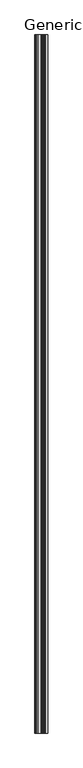
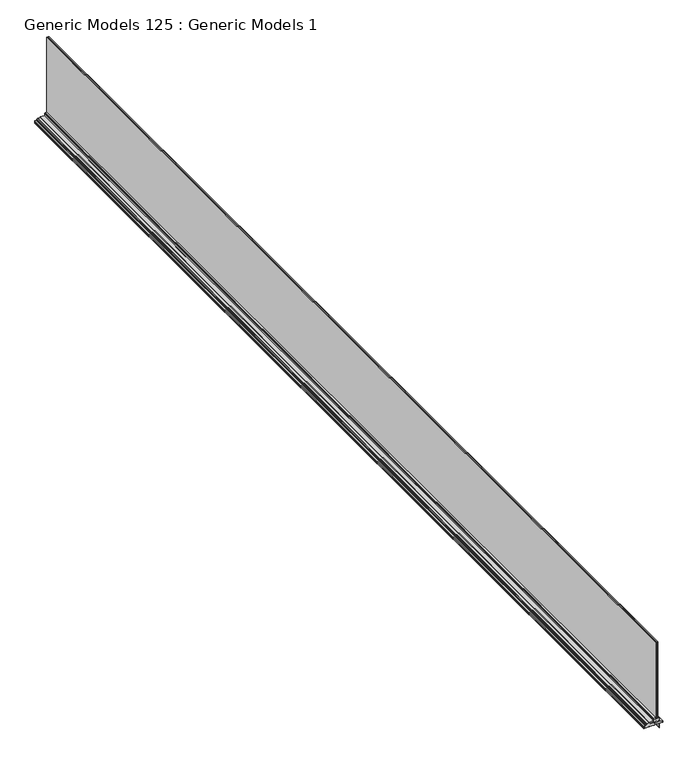
"""IFC4 building model written with IfcOpenShell, lengths in millimetres: proxy geometry, Generic Models 125 : Generic Models 1."""

from ifc_helpers import new_model, si_unit, point, frame, frame_2d, origin, place, context, project, spatial, polyline, circle_curve, trimmed, segment, composite_curve, outline, extrude, source, transform, mapped, element, save


def generic_models_125_generic_models_1_b7fb5337(model_context):
    return source(origin(), model_context, "Body", "SweptSolid", [
        extrude(outline(composite_curve([segment(polyline([(126266.1189906, 4830.4400913), (126266.1189906, 4848.5086347), (126269.2939906, 4848.5086347), (126269.2939906, 4850.7946386), (126266.1189906, 4850.7946386), (126266.1189906, 4868.3023877), (126269.2939906, 4868.3023877), (126269.2939906, 4870.5883916), (126266.1189906, 4870.5883916), (126266.1189906, 4887.6154913), (126268.2017906, 4887.6154913), (126268.2017906, 4890.7904913), (126266.1189906, 4890.7904913), (126266.1189906, 4907.8898738), (126269.2939906, 4907.8898738), (126269.2939906, 4910.1758738), (126266.1189906, 4910.1758738), (126266.1189906, 4946.6450416), (126230.747103, 4946.6450416)]), True, "CONTINUOUS"), segment(trimmed(circle_curve(frame_2d((126230.7494439, 4947.3435419)), 0.6985041), [point((126230.747103, 4946.6450416))], [point((126230.7519036, 4948.0420416))], False, "CARTESIAN"), True, "CONTINUOUS"), segment(polyline([(126230.7519036, 4948.0420416), (126266.1189906, 4948.0420416), (126266.1189906, 4972.929876), (126267.5159906, 4972.929876), (126267.5159906, 4966.579876), (126269.8019906, 4966.579876), (126269.8019906, 4974.4834416), (126278.7334139, 4974.4834416), (126281.1557838, 4946.6196416), (126281.1557838, 4911.6692416), (126286.0325764, 4911.6692416), (126286.0325764, 4907.6561145), (126279.6136368, 4907.6561145), (126279.6136368, 4905.6748401), (126287.5638299, 4905.6748401), (126287.5638299, 4897.2675044), (126288.5036264, 4897.2675044), (126288.5036264, 4879.7415044), (126290.7896264, 4879.7415044), (126290.7896264, 4897.2675044), (126299.4764264, 4897.2675044), (126299.4764264, 4900.3154773), (126302.6514264, 4900.3154773), (126302.6514264, 4870.9022533), (126296.3195939, 4870.9022533), (126296.3195939, 4851.8522533), (126293.9319974, 4851.8522533), (126293.9319974, 4850.2520602), (126290.7569974, 4846.3150913), (126290.7569974, 4844.7148982), (126286.7945939, 4844.7148982), (126286.7945939, 4841.5398982), (126285.9818043, 4840.7524463), (126285.9818043, 4830.4400913), (126276.0503853, 4830.4400913), (126276.0503853, 4838.3902843), (126274.0692078, 4838.3902843), (126274.0692078, 4830.4400913), (126266.1189906, 4830.4400913)]), True, "CONTINUOUS")], self_intersect=False)), frame((0.0, -1504.2676118, 0.0), z_axis=(0.0, 1.0, 0.0), x_axis=(0.0, 0.0, 1.0)), (0.0, 0.0, 1.0), 7886.7),
        extrude(outline(composite_curve([segment(polyline([(126314.9759014, 4938.1431837), (126313.9527594, 4937.1200416), (126310.3721406, 4937.1200416), (126310.3721406, 4915.6826708), (126312.7604294, 4918.0709596), (126322.6918294, 4918.0709596), (126321.6791794, 4906.2432791), (126319.5168294, 4906.2432791), (126319.5168294, 4902.4753596), (126311.9730294, 4902.4753596), (126311.9730294, 4904.0755596), (126310.3721406, 4904.0755596), (126310.3721406, 4902.1950416), (126292.0841406, 4902.1950416)]), True, "CONTINUOUS"), segment(trimmed(circle_curve(frame_2d((126292.0841406, 4903.0078416)), 0.8128), [point((126292.0841406, 4902.1950416))], [point((126291.2713406, 4903.0078416))], False, "CARTESIAN"), True, "CONTINUOUS"), segment(polyline([(126291.2713406, 4903.0078416), (126291.2713406, 4916.3428416)]), True, "CONTINUOUS"), segment(trimmed(circle_curve(frame_2d((126291.2713406, 4918.3240416)), 1.9812), [point((126291.2713406, 4916.3428416))], [point((126291.2713406, 4920.3052416))], True, "CARTESIAN"), True, "CONTINUOUS"), segment(polyline([(126291.2713406, 4920.3052416), (126291.2713406, 4932.4972416), (126285.9627406, 4932.4972416), (126285.9627406, 4938.1106416), (126293.8875406, 4938.1106416), (126293.8875406, 4940.0156416), (126290.5855406, 4940.0156416), (126290.5855406, 4941.6920416), (126288.5535406, 4941.6920416), (126288.5535406, 4944.2574416)]), True, "CONTINUOUS"), segment(trimmed(circle_curve(frame_2d((126290.9411406, 4944.2574416)), 2.3876), [point((126288.5535406, 4944.2574416))], [point((126290.9411406, 4946.6450416))], False, "CARTESIAN"), True, "CONTINUOUS"), segment(polyline([(126290.9411406, 4946.6450416), (126313.2423406, 4946.6450416), (126313.2423406, 4944.2574416), (126321.0481641, 4941.7220811), (126321.2377144, 4939.2790416), (126319.2113406, 4939.2790416), (126319.2113406, 4938.1431837), (126314.9759014, 4938.1431837)]), True, "CONTINUOUS")], self_intersect=False)), frame((0.0, -1504.2676118, 0.0), z_axis=(0.0, 1.0, 0.0), x_axis=(0.0, 0.0, 1.0)), (0.0, 0.0, 1.0), 7886.7),
        extrude(outline(polyline([(4923.6272096, -1504.2676118), (4918.8647096, -1504.2676118), (4918.8647096, 6382.4323882), (4923.6272096, 6382.4323882), (4923.6272096, -1504.2676118)])), frame((0.0, 0.0, 126311.1658906), z_axis=(0.0, 0.0, 1.0), x_axis=(1.0, 0.0, 0.0)), (0.0, 0.0, 1.0), 602.3375481),
        extrude(outline(polyline([(4930.7700416, -1504.2676118), (4924.4209596, -1504.2676118), (4924.4209596, 6382.4323882), (4930.7700416, 6382.4323882), (4930.7700416, -1504.2676118)])), frame((0.0, 0.0, 126311.1658906), z_axis=(0.0, 0.0, 1.0), x_axis=(1.0, 0.0, 0.0)), (0.0, 0.0, 1.0), 6.35),
        extrude(outline(polyline([(4936.3262916, -1504.2676118), (4931.5637916, -1504.2676118), (4931.5637916, 6382.4323882), (4936.3262916, 6382.4323882), (4936.3262916, -1504.2676118)])), frame((0.0, 0.0, 126311.1658906), z_axis=(0.0, 0.0, 1.0), x_axis=(1.0, 0.0, 0.0)), (0.0, 0.0, 1.0), 602.3375481),
    ])


if __name__ == "__main__":
    model = new_model("IFC4")
    model_context = context("Model", 3, world=origin())
    ifc_project = project(units=[si_unit("LENGTHUNIT", "METRE", prefix="MILLI")], contexts=[model_context])
    site = spatial("IfcSite", under=ifc_project)
    building = spatial("IfcBuilding", under=site)
    placement = place(None, origin())
    generic_models_125_generic_models_1_shape = generic_models_125_generic_models_1_b7fb5337(model_context)
    element("IfcBuildingElementProxy", 1, Name="Generic Models 125 : Generic Models 1", ObjectType="Generic Models 125 : Generic Models 1", at=placement, inside=building, context=model_context, shape_type="MappedRepresentation", body=[
        mapped(generic_models_125_generic_models_1_shape, transform((0.0, 0.0, 0.0), x_axis=(1.0, 0.0, 0.0), y_axis=(0.0, 1.0, 0.0), z_axis=(0.0, 0.0, 1.0))),
    ])
    save(model, "model.ifc")

# Revit data of these elements
# Element 1 (IfcBuildingElementProxy, "Generic Models 125 : Generic Models 1")
#   Materials on its faces: "_WINDOW PER SCHEDULE"
# Materials
#   "_WINDOW PER SCHEDULE": class "Generic", colour RGB 255 255 255, transparency 0, Cost = 0
